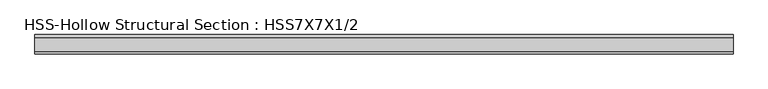
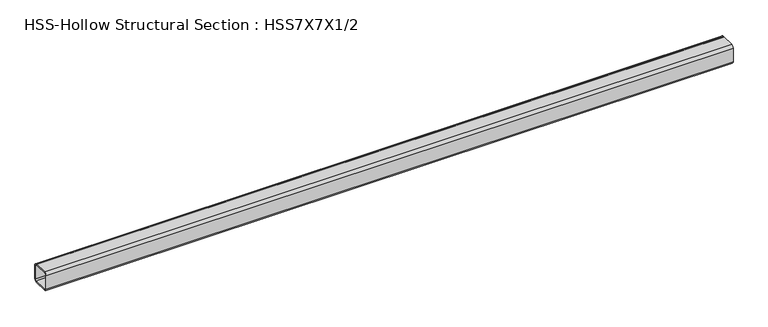
"""IFC4 building model written with IfcOpenShell, lengths in millimetres: member geometry, HSS-Hollow Structural Section : HSS7X7X1/2."""

from ifc_helpers import new_model, si_unit, point, frame, frame_2d, origin, place, context, project, spatial, polyline, circle_curve, trimmed, segment, composite_curve, outline, extrude, source, transform, mapped, element, save


def hss_hollow_structural_section_hss7x7x1_2_4e5f93a8(model_context):
    return source(origin(), model_context, "Body", "SweptSolid", [
        extrude(outline(composite_curve([segment(polyline([(88.9, 65.278), (88.9, -65.278)]), True, "CONTINUOUS"), segment(trimmed(circle_curve(frame_2d((65.278, -65.278)), 23.622), [point((88.9, -65.278))], [point((65.278, -88.9))], False, "CARTESIAN"), True, "CONTINUOUS"), segment(polyline([(65.278, -88.9), (-65.278, -88.9)]), True, "CONTINUOUS"), segment(trimmed(circle_curve(frame_2d((-65.278, -65.278)), 23.622), [point((-65.278, -88.9))], [point((-88.9, -65.278))], False, "CARTESIAN"), True, "CONTINUOUS"), segment(polyline([(-88.9, -65.278), (-88.9, 65.278)]), True, "CONTINUOUS"), segment(trimmed(circle_curve(frame_2d((-65.278, 65.278)), 23.622), [point((-88.9, 65.278))], [point((-65.278, 88.9))], False, "CARTESIAN"), True, "CONTINUOUS"), segment(polyline([(-65.278, 88.9), (65.278, 88.9)]), True, "CONTINUOUS"), segment(trimmed(circle_curve(frame_2d((65.278, 65.278)), 23.622), [point((65.278, 88.9))], [point((88.9, 65.278))], False, "CARTESIAN"), True, "CONTINUOUS")], self_intersect=False), holes=[composite_curve([segment(trimmed(circle_curve(frame_2d((-65.278, 65.278)), 11.811), [point((-65.278, 77.089))], [point((-77.089, 65.278))], True, "CARTESIAN"), True, "CONTINUOUS"), segment(polyline([(-77.089, 65.278), (-77.089, -65.278)]), True, "CONTINUOUS"), segment(trimmed(circle_curve(frame_2d((-65.278, -65.278)), 11.811), [point((-77.089, -65.278))], [point((-65.278, -77.089))], True, "CARTESIAN"), True, "CONTINUOUS"), segment(polyline([(-65.278, -77.089), (65.278, -77.089)]), True, "CONTINUOUS"), segment(trimmed(circle_curve(frame_2d((65.278, -65.278)), 11.811), [point((65.278, -77.089))], [point((77.089, -65.278))], True, "CARTESIAN"), True, "CONTINUOUS"), segment(polyline([(77.089, -65.278), (77.089, 65.278)]), True, "CONTINUOUS"), segment(trimmed(circle_curve(frame_2d((65.278, 65.278)), 11.811), [point((77.089, 65.278))], [point((65.278, 77.089))], True, "CARTESIAN"), True, "CONTINUOUS"), segment(polyline([(65.278, 77.089), (-65.278, 77.089)]), True, "CONTINUOUS")], self_intersect=False)]), frame((-2916.3739489, 0.0, 0.0), z_axis=(1.0, 0.0, 0.0), x_axis=(0.0, 1.0, 0.0)), (0.0, 0.0, 1.0), 6360.5683713),
    ])


if __name__ == "__main__":
    model = new_model("IFC4")
    model_context = context("Model", 3, world=origin())
    ifc_project = project(units=[si_unit("LENGTHUNIT", "METRE", prefix="MILLI")], contexts=[model_context])
    site = spatial("IfcSite", under=ifc_project)
    building = spatial("IfcBuilding", under=site)
    placement = place(None, origin())
    hss_hollow_structural_section_hss7x7x1_2_shape = hss_hollow_structural_section_hss7x7x1_2_4e5f93a8(model_context)
    element("IfcMember", 1, ObjectType="HSS-Hollow Structural Section : HSS7X7X1/2", at=placement, inside=building, context=model_context, shape_type="MappedRepresentation", body=[
        mapped(hss_hollow_structural_section_hss7x7x1_2_shape, transform((0.0, 0.0, 0.0), x_axis=(1.0, 0.0, 0.0), y_axis=(0.0, 1.0, 0.0), z_axis=(0.0, 0.0, 1.0))),
    ])
    save(model, "model.ifc")

# Revit data of these elements
# Type "HSS-Hollow Structural Section : HSS7X7X1/2"
#   Assembly Code = "B10"
#   Shape = "Square"
#   W = 41.9
#   Ht = 0' - 7"
#   Length [instance default] = 5' - 0"
#   b = 0' - 7"
#   kr = 0' - 0.93"
#   t = 0' - 0.465"
#   A = 0.0805556 SF
#   Structural Material [instance default] = Steel ASTM A500, Grade B, Rectangular and Square
# Element 1 (IfcMember, "HSS-Hollow Structural Section : HSS7X7X1/2")
#   Materials on its faces: "Steel ASTM A500, Grade B, Rectangular and Square"
# Materials
#   "Steel ASTM A500, Grade B, Rectangular and Square": class "Metal", colour RGB 199 199 199, transparency 0, Description = "Carbon steel", Cost = 0
